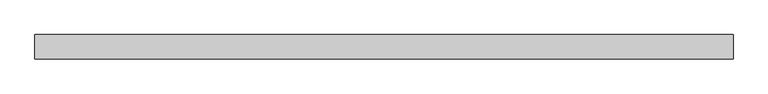
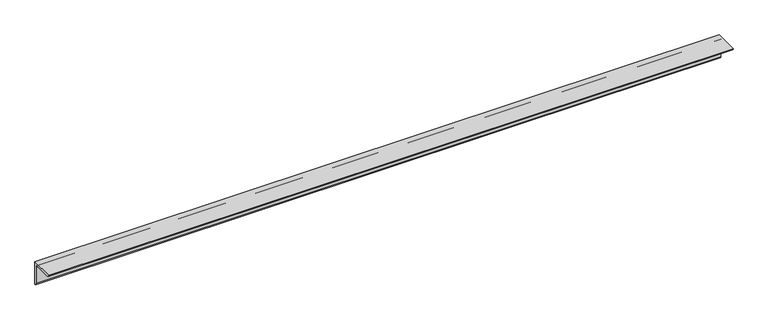
"""IFC4 building model written with IfcOpenShell, lengths in millimetres: member geometry, 0912_Steel Framing_L-KSD3502 : H_SB_AR_S03_L-130x130x12_HBR3."""

from ifc_helpers import new_model, si_unit, point, frame, frame_2d, origin, place, context, project, spatial, polyline, circle_curve, trimmed, segment, composite_curve, outline, extrude, source, transform, mapped, element, save


def member_c049ea03(model_context):
    return source(origin(), model_context, "Body", "SweptSolid", [
        extrude(outline(composite_curve([segment(polyline([(36.4, 36.4), (36.4, -93.6)]), True, "CONTINUOUS"), segment(trimmed(circle_curve(frame_2d((36.4, -81.6)), 12.0), [point((36.4, -93.6))], [point((24.4, -81.6))], False, "CARTESIAN"), True, "CONTINUOUS"), segment(polyline([(24.4, -81.6), (24.4, 12.4)]), True, "CONTINUOUS"), segment(trimmed(circle_curve(frame_2d((12.4, 12.4)), 12.0), [point((24.4, 12.4))], [point((12.4, 24.4))], True, "CARTESIAN"), True, "CONTINUOUS"), segment(polyline([(12.4, 24.4), (-81.6, 24.4)]), True, "CONTINUOUS"), segment(trimmed(circle_curve(frame_2d((-81.6, 36.4)), 12.0), [point((-81.6, 24.4))], [point((-93.6, 36.4))], False, "CARTESIAN"), True, "CONTINUOUS"), segment(polyline([(-93.6, 36.4), (36.4, 36.4)]), True, "CONTINUOUS")], self_intersect=False)), frame((-1867.6865023, 0.0, 0.0), z_axis=(1.0, 0.0, 0.0), x_axis=(0.0, 1.0, 0.0)), (0.0, 0.0, 1.0), 3720.541926),
    ])


if __name__ == "__main__":
    model = new_model("IFC4")
    model_context = context("Model", 3, world=origin())
    ifc_project = project(units=[si_unit("LENGTHUNIT", "METRE", prefix="MILLI")], contexts=[model_context])
    site = spatial("IfcSite", under=ifc_project)
    building = spatial("IfcBuilding", under=site)
    placement = place(None, origin())
    member_shape = member_c049ea03(model_context)
    element("IfcMember", 1, ObjectType="0912_Steel Framing_L-KSD3502 : H_SB_AR_S03_L-130x130x12_HBR3", at=placement, inside=building, context=model_context, shape_type="MappedRepresentation", body=[
        mapped(member_shape, transform((0.0, 0.0, 0.0), x_axis=(1.0, 0.0, 0.0), y_axis=(0.0, 1.0, 0.0), z_axis=(0.0, 0.0, 1.0))),
    ])
    save(model, "model.ifc")

# Revit data of these elements
# Type "0912_Steel Framing_L-KSD3502 : H_SB_AR_S03_L-130x130x12_HBR3"
#   k = 25 mm
#   Perimeter = 0.52 m²/m
#   Nominal Weight = 23.40 kgf/m
#   Length [instance default] = 1000 mm
#   b = 130 mm
#   d = 130 mm
#   t = 12 mm
#   x = 36.4 mm
#   y = 36.4 mm
#   A = 2976.00 m²
#   Structural Material [instance default] = Steel, 45-345
# Element 1 (IfcMember, "0912_Steel Framing_L-KSD3502 : H_SB_AR_S03_L-130x130x12_HBR3")
#   Materials on its faces: "Steel, 45-345"
# Materials
#   "Steel, 45-345": class "Metal", colour RGB 189 187 185, transparency 0, Description = "Steel 345 MPa", Cost = 0
